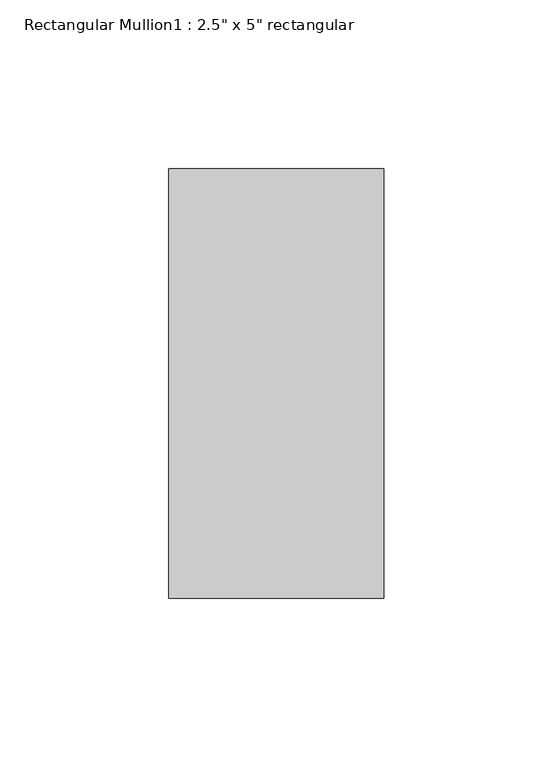
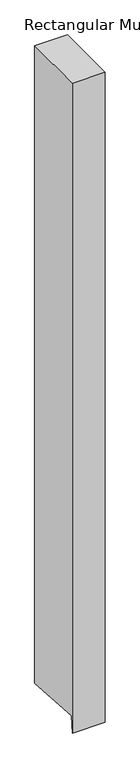
"""IFC4 building model written with IfcOpenShell, lengths in millimetres: member geometry."""

import ifcopenshell
import ifcopenshell.guid

model = None  # the IFC model being written
_history = None  # IfcOwnerHistory: only IFC2X3 demands one
_inside = {}  # id of a spatial element -> (the spatial element, [elements in it])
_under = {}  # id of a project, library or spatial element -> (it, [spatial elements below it])
_declared = {}  # id of a project -> (the project, [libraries it declares])
_typed = {}  # id of a type object -> (the type object, [elements of that type])
_made_of = {}  # id of a material, layer set ... -> (it, [elements and type objects made of it])


def new_model(schema):
    """Start an empty IFC model of exactly this schema.

    Asked for "IFC4X3", IfcOpenShell would pick the latest addendum, in which some entities
    have other attributes; the version numbers below select the first issue.
    IFC2X3 requires an IfcOwnerHistory on every rooted entity: one is made here for all.
    """
    global model, _history
    if schema == "IFC4X3":
        model = ifcopenshell.file(schema_version=(4, 3, 0, 0))
    else:
        model = ifcopenshell.file(schema=schema)
    _inside.clear()
    _under.clear()
    _declared.clear()
    _typed.clear()
    _made_of.clear()
    _history = None
    if model.schema == "IFC2X3":
        org = make("IfcOrganization", Name="unknown")
        user = make(
            "IfcPersonAndOrganization",
            ThePerson=make("IfcPerson", FamilyName="unknown"),
            TheOrganization=org,
        )
        app = make(
            "IfcApplication",
            ApplicationDeveloper=org,
            Version="unknown",
            ApplicationFullName="unknown",
            ApplicationIdentifier="unknown",
        )
        _history = make(
            "IfcOwnerHistory",
            OwningUser=user,
            OwningApplication=app,
            ChangeAction="ADDED",
            CreationDate=0,
        )
    return model


def make(cls, **values):
    """One entity of the class cls with the attributes given. An attribute that is None is left unset."""
    return model.create_entity(
        cls, **{name: value for name, value in values.items() if value is not None}
    )


def rooted(cls, **values):
    """An entity with a GlobalId (a new one), such as an element, a storey or a relation."""
    return make(cls, GlobalId=ifcopenshell.guid.new(), OwnerHistory=_history, **values)


def si_unit(unit_type, name, prefix=None):
    """IfcSIUnit, for example si_unit("LENGTHUNIT", "METRE", prefix="MILLI")."""
    return make("IfcSIUnit", UnitType=unit_type, Prefix=prefix, Name=name)


def assignment(units):
    """IfcUnitAssignment: the units of a project."""
    return None if units is None else make("IfcUnitAssignment", Units=units)


def point(xyz):
    """IfcCartesianPoint."""
    return None if xyz is None else make("IfcCartesianPoint", Coordinates=xyz)


def direction(xyz):
    """IfcDirection."""
    return None if xyz is None else make("IfcDirection", DirectionRatios=xyz)


def frame(location, z_axis=None, x_axis=None):
    """IfcAxis2Placement3D, a coordinate frame: its origin and axes. An axis left out is left unset."""
    return make(
        "IfcAxis2Placement3D",
        Location=point(location),
        Axis=direction(z_axis),
        RefDirection=direction(x_axis),
    )


def origin():
    """The frame at (0, 0, 0) with its axes left unset."""
    return frame((0.0, 0.0, 0.0))


def place(relative_to, where):
    """IfcLocalPlacement: puts the frame where relative to a parent placement (None: the world)."""
    return make(
        "IfcLocalPlacement", PlacementRelTo=relative_to, RelativePlacement=where
    )


def context(
    kind, dimensions, precision=None, world=None, true_north=None, identifier=None
):
    """IfcGeometricRepresentationContext, for example the 3D "Model" context."""
    return make(
        "IfcGeometricRepresentationContext",
        ContextIdentifier=identifier,
        ContextType=kind,
        CoordinateSpaceDimension=dimensions,
        Precision=precision,
        WorldCoordinateSystem=world,
        TrueNorth=true_north,
    )


def project(units=None, contexts=None):
    """IfcProject with its units and contexts."""
    return rooted(
        "IfcProject",
        Name="project",
        RepresentationContexts=contexts,
        UnitsInContext=assignment(units),
    )


def spatial(cls, under=None, at=None, **own):
    """A site, building, storey or space (cls), placed at a placement, below another one or the project."""
    s = rooted(cls, ObjectPlacement=at, **own)
    if under is not None:
        _under.setdefault(under.id(), (under, []))[1].append(s)
    return s


def polyline(points):
    """IfcPolyline through the points."""
    return make("IfcPolyline", Points=[point(p) for p in points])


def outline(outer, holes=None, kind="AREA"):
    """IfcArbitraryClosedProfileDef: a profile drawn as a closed curve; with holes, ...WithVoids."""
    if holes is None:
        return make("IfcArbitraryClosedProfileDef", ProfileType=kind, OuterCurve=outer)
    return make(
        "IfcArbitraryProfileDefWithVoids",
        ProfileType=kind,
        OuterCurve=outer,
        InnerCurves=holes,
    )


def extrude(swept, where, along, depth):
    """IfcExtrudedAreaSolid: the profile swept, set in the frame where, extruded along a direction by depth."""
    return make(
        "IfcExtrudedAreaSolid",
        SweptArea=swept,
        Position=where,
        ExtrudedDirection=direction(along),
        Depth=depth,
    )


def shape(context_of_items, identifier, shape_type, items):
    """IfcShapeRepresentation: the items that make up one representation, for example the "Body"."""
    return make(
        "IfcShapeRepresentation",
        ContextOfItems=context_of_items,
        RepresentationIdentifier=identifier,
        RepresentationType=shape_type,
        Items=items,
    )


def source(mapping_origin, context_of_items, identifier, shape_type, items):
    """IfcRepresentationMap: a shape defined once, which mapped items show again and again."""
    return make(
        "IfcRepresentationMap",
        MappingOrigin=mapping_origin,
        MappedRepresentation=shape(context_of_items, identifier, shape_type, items),
    )


def transform(
    local_origin,
    x_axis=None,
    y_axis=None,
    z_axis=None,
    scale=None,
    scale2=None,
    scale3=None,
    uniform=True,
):
    """IfcCartesianTransformationOperator3D, or its non-uniform kind. x_axis, y_axis, z_axis: its Axis1, 2, 3."""
    if uniform:
        return make(
            "IfcCartesianTransformationOperator3D",
            Axis1=direction(x_axis),
            Axis2=direction(y_axis),
            LocalOrigin=point(local_origin),
            Scale=scale,
            Axis3=direction(z_axis),
        )
    return make(
        "IfcCartesianTransformationOperator3DnonUniform",
        Axis1=direction(x_axis),
        Axis2=direction(y_axis),
        LocalOrigin=point(local_origin),
        Scale=scale,
        Axis3=direction(z_axis),
        Scale2=scale2,
        Scale3=scale3,
    )


def mapped(mapping_source, mapping_target):
    """IfcMappedItem: shows the shape of a source again, moved by a transform."""
    return make(
        "IfcMappedItem", MappingSource=mapping_source, MappingTarget=mapping_target
    )


def made_of(thing, what):
    """Note that an element or type object is made of a material, layer set ...; save() writes the relation."""
    if what is not None:
        _made_of.setdefault(what.id(), (what, []))[1].append(thing)
    return thing


def element(
    cls,
    number,
    at=None,
    inside=None,
    cuts=None,
    type_object=None,
    material=None,
    context=None,
    identifier="Body",
    shape_type=None,
    held_by="IfcProductDefinitionShape",
    body=None,
    shapes=None,
    **own,
):
    """One element of the class cls, such as IfcWall. Its Tag is "e" and its number.

    at: its placement. inside: the storey or other place that contains it. cuts: it is an
    opening in that element (IfcRelVoidsElement). A single representation is given by context,
    identifier, shape_type and body (its items); several are given by shapes. held_by: the class
    of the entity that holds the representations. save() writes the other relations.
    """
    e = rooted(cls, Tag="e%d" % number, ObjectPlacement=at, **own)
    if body is not None:
        shapes = [shape(context, identifier, shape_type, body)]
    if shapes is not None:
        e.Representation = make(held_by, Representations=shapes)
    if inside is not None:
        _inside.setdefault(inside.id(), (inside, []))[1].append(e)
    if cuts is not None:
        rooted(
            "IfcRelVoidsElement", RelatingBuildingElement=cuts, RelatedOpeningElement=e
        )
    if type_object is not None:
        _typed.setdefault(type_object.id(), (type_object, []))[1].append(e)
    return made_of(e, material)


def aggregate(whole, parts):
    """IfcRelAggregates: a whole, such as a stair, and the parts it consists of."""
    return rooted("IfcRelAggregates", RelatingObject=whole, RelatedObjects=parts)


def save(model, path):
    """Write the relations noted so far, then the file.

    IfcRelAggregates (storeys below a building ...), IfcRelContainedInSpatialStructure (elements
    in a storey), IfcRelDefinesByType, IfcRelAssociatesMaterial and IfcRelDeclares: one each for
    every whole, place, type object, material and project.
    """
    for whole, parts in _under.values():
        aggregate(whole, parts)
    for where, things in _inside.values():
        rooted(
            "IfcRelContainedInSpatialStructure",
            RelatedElements=things,
            RelatingStructure=where,
        )
    for kind, things in _typed.values():
        rooted("IfcRelDefinesByType", RelatedObjects=things, RelatingType=kind)
    for what, things in _made_of.values():
        rooted("IfcRelAssociatesMaterial", RelatedObjects=things, RelatingMaterial=what)
    for by, libraries in _declared.values():
        rooted("IfcRelDeclares", RelatingContext=by, RelatedDefinitions=libraries)
    model.write(path)


def member_1ee05d72(model_context):
    return source(origin(), model_context, "Body", "SweptSolid", [
        extrude(outline(polyline([(-63.5, 0.0), (63.5, 0.0), (63.5, -1307.2809876), (-61.0425175, -1298.2675313), (-63.5, -1332.2235469), (-63.5, 0.0)])), frame((-63.5, 0.0, 0.0), z_axis=(1.0, 0.0, 0.0), x_axis=(0.0, 1.0, 0.0)), (0.0, 0.0, 1.0), 63.5),
    ])


if __name__ == "__main__":
    model = new_model("IFC4")
    model_context = context("Model", 3, world=origin())
    ifc_project = project(units=[si_unit("LENGTHUNIT", "METRE", prefix="MILLI")], contexts=[model_context])
    site = spatial("IfcSite", under=ifc_project)
    building = spatial("IfcBuilding", under=site)
    placement = place(None, origin())
    member_shape = member_1ee05d72(model_context)
    element("IfcMember", 1, ObjectType="Rectangular Mullion1 : 2.5\" x 5\" rectangular", at=placement, inside=building, context=model_context, shape_type="MappedRepresentation", body=[
        mapped(member_shape, transform((0.0, 0.0, 0.0), x_axis=(1.0, 0.0, 0.0), y_axis=(0.0, 1.0, 0.0), z_axis=(0.0, 0.0, 1.0))),
    ])
    save(model, "model.ifc")

# Revit data of these elements
# Type "Rectangular Mullion1 : 2.5\" x 5\" rectangular"
#   built-in parameter 1007304 = 0.416667 (stored number, unit not read)
#   built-in parameter 1007301 = 0.104167 (stored number, unit not read)
#   built-in parameter 1007300 = 0.104167 (stored number, unit not read)
# Element 1 (IfcMember, "Rectangular Mullion1 : 2.5\" x 5\" rectangular")
#   Materials on its faces: "support-frame"
# Materials
#   "support-frame": class "Unassigned", colour RGB 233 233 233, transparency 0, Cost = 0
